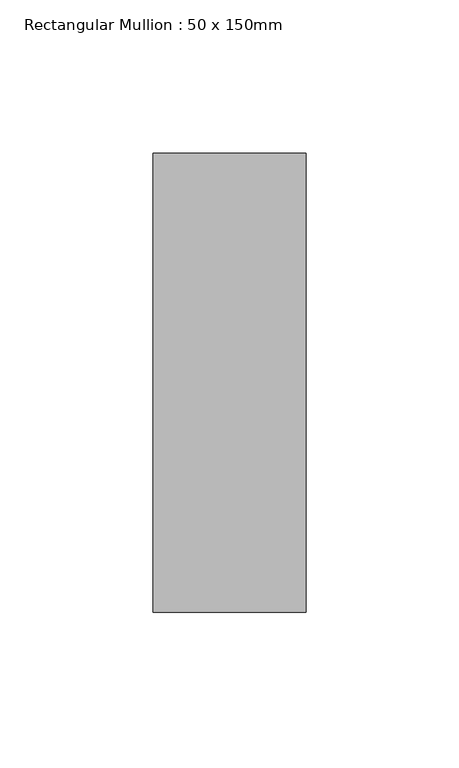
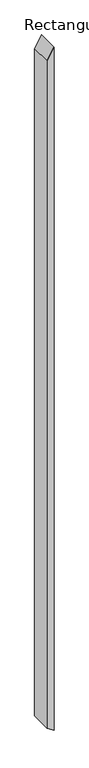
"""IFC4 building model written with IfcOpenShell, lengths in millimetres: member geometry, Rectangular Mullion : 50 x 150mm."""

from ifc_helpers import new_model, si_unit, frame, origin, place, context, project, spatial, polyline, outline, extrude, source, transform, mapped, element, save


def rectangular_mullion_50_x_150mm_5700b0c8(model_context):
    return source(origin(), model_context, "Body", "SweptSolid", [
        extrude(outline(polyline([(0.0, 0.0), (-86.4378444, -50.0), (-5081.8724884, -50.0), (-5115.611673, 0.0), (0.0, 0.0)])), frame((0.0, -75.0, 0.0), z_axis=(0.0, 1.0, 0.0), x_axis=(0.0, 0.0, 1.0)), (0.0, 0.0, 1.0), 150.0),
    ])


if __name__ == "__main__":
    model = new_model("IFC4")
    model_context = context("Model", 3, world=origin())
    ifc_project = project(units=[si_unit("LENGTHUNIT", "METRE", prefix="MILLI")], contexts=[model_context])
    site = spatial("IfcSite", under=ifc_project)
    building = spatial("IfcBuilding", under=site)
    placement = place(None, origin())
    rectangular_mullion_50_x_150mm_shape = rectangular_mullion_50_x_150mm_5700b0c8(model_context)
    element("IfcMember", 1, ObjectType="Rectangular Mullion : 50 x 150mm", at=placement, inside=building, context=model_context, shape_type="MappedRepresentation", body=[
        mapped(rectangular_mullion_50_x_150mm_shape, transform((0.0, 0.0, 0.0), x_axis=(1.0, 0.0, 0.0), y_axis=(0.0, 1.0, 0.0), z_axis=(0.0, 0.0, 1.0))),
    ])
    save(model, "model.ifc")

# Revit data of these elements
# Type "Rectangular Mullion : 50 x 150mm"
#   built-in parameter 1007304 = 0.492126 (stored number, unit not read)
#   built-in parameter 1007301 = 0.082021 (stored number, unit not read)
#   built-in parameter 1007300 = 0.082021 (stored number, unit not read)
# Element 1 (IfcMember, "Rectangular Mullion : 50 x 150mm")
#   Materials on its faces: "Metal - Aluminium"
# Materials
#   "Metal - Aluminium": class "Metal", colour RGB 247 247 247, transparency 0
